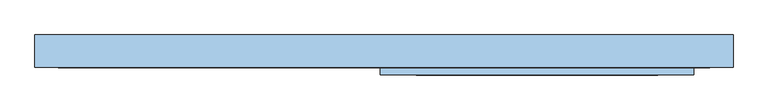
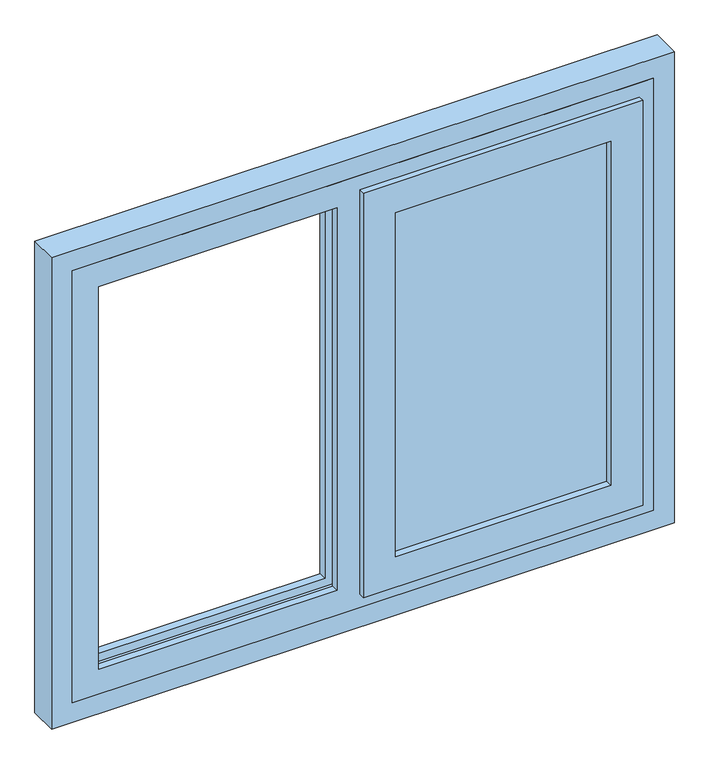
"""IFC4 building model written with IfcOpenShell, lengths in millimetres: window geometry, Окно 2-Откидное - Левое глухое - Один переплет с многокамерным стеклопакетом - 30674-99 : ОП Г1  1160-1470 (4M1-10-4M1-10-4M1) ГОСТ 30674-99."""

from ifc_helpers import new_model, si_unit, frame, origin, place, context, project, spatial, polyline, outline, extrude, faceted_brep, source, transform, mapped, element, save


def window_999542c6(model_context):
    return source(origin(), model_context, "Body", "SolidModel", [
        extrude(outline(polyline([(942.0, 608.0), (1858.0, 608.0), (1858.0, 49.0), (942.0, 49.0), (942.0, 608.0)]), holes=[polyline([(1843.0, 593.0), (957.0, 593.0), (957.0, 64.0), (1843.0, 64.0), (1843.0, 593.0)])]), frame((0.0, 25.0, 0.0), z_axis=(0.0, 1.0, 0.0), x_axis=(0.0, 0.0, 1.0)), (0.0, 0.0, 1.0), 10.0),
        extrude(outline(polyline([(942.0, 608.0), (1858.0, 608.0), (1858.0, 49.0), (942.0, 49.0), (942.0, 608.0)]), holes=[polyline([(1843.0, 593.0), (957.0, 593.0), (957.0, 64.0), (1843.0, 64.0), (1843.0, 593.0)])]), frame((0.0, 11.0, 0.0), z_axis=(0.0, 1.0, 0.0), x_axis=(0.0, 0.0, 1.0)), (0.0, 0.0, 1.0), 10.0),
        extrude(outline(polyline([(49.0, 25.0), (608.0, 25.0), (608.0, 21.0), (49.0, 21.0), (49.0, 25.0)])), frame((0.0, 0.0, 942.0), z_axis=(0.0, 0.0, 1.0), x_axis=(1.0, 0.0, 0.0)), (0.0, 0.0, 1.0), 916.0),
        extrude(outline(polyline([(49.0, 39.0), (608.0, 39.0), (608.0, 35.0), (49.0, 35.0), (49.0, 39.0)])), frame((0.0, 0.0, 942.0), z_axis=(0.0, 0.0, 1.0), x_axis=(1.0, 0.0, 0.0)), (0.0, 0.0, 1.0), 916.0),
        extrude(outline(polyline([(49.0, 11.0), (608.0, 11.0), (608.0, 7.0), (49.0, 7.0), (49.0, 11.0)])), frame((0.0, 0.0, 942.0), z_axis=(0.0, 0.0, 1.0), x_axis=(1.0, 0.0, 0.0)), (0.0, 0.0, 1.0), 916.0),
        faceted_brep([(-700.0, 5.0, 1950.0), (-700.0, 75.0, 1950.0), (-700.0, 75.0, 850.0), (-700.0, 5.0, 850.0), (700.0, 75.0, 850.0), (700.0, 75.0, 1950.0), (-637.0, 75.0, 1887.0), (-637.0, 75.0, 913.0), (-63.0, 75.0, 913.0), (-63.0, 75.0, 1887.0), (19.0, 75.0, 1887.0), (19.0, 75.0, 913.0), (637.0, 75.0, 913.0), (637.0, 75.0, 1887.0), (700.0, 5.0, 850.0), (700.0, 5.0, 1950.0), (-637.0, 5.0, 913.0), (-637.0, 5.0, 1887.0), (-63.0, 5.0, 1887.0), (-63.0, 5.0, 913.0), (0.0, 5.0, 893.0), (0.0, 5.0, 1907.0), (657.0, 5.0, 1907.0), (657.0, 5.0, 893.0), (-637.0, 23.0, 1887.0), (-637.0, 23.0, 913.0), (-63.0, 23.0, 913.0), (-657.0, 23.0, 893.0), (-657.0, 23.0, 1907.0), (-43.0, 23.0, 1907.0), (-43.0, 23.0, 893.0), (-63.0, 23.0, 1887.0), (-657.0, 55.0, 1907.0), (-657.0, 55.0, 893.0), (-43.0, 55.0, 893.0), (-43.0, 55.0, 1907.0), (-637.0, 55.0, 913.0), (-637.0, 55.0, 1887.0), (-63.0, 55.0, 1887.0), (-63.0, 55.0, 913.0), (0.0, 61.0, 893.0), (0.0, 61.0, 1907.0), (657.0, 61.0, 893.0), (657.0, 61.0, 1907.0), (19.0, 61.0, 913.0), (19.0, 61.0, 1887.0), (637.0, 61.0, 1887.0), (637.0, 61.0, 913.0)], [[[0, 1, 2, 3]], [[4, 2, 1, 5], [6, 7, 8, 9], [10, 11, 12, 13]], [[3, 2, 4, 14]], [[15, 0, 3, 14], [16, 17, 18, 19], [20, 21, 22, 23]], [[24, 17, 16, 25]], [[25, 16, 19, 26]], [[27, 28, 29, 30], [24, 25, 26, 31]], [[32, 28, 27, 33]], [[33, 27, 30, 34]], [[32, 33, 34, 35], [36, 37, 38, 39]], [[6, 37, 36, 7]], [[7, 36, 39, 8]], [[15, 14, 4, 5]], [[26, 19, 18, 31]], [[34, 30, 29, 35]], [[8, 39, 38, 9]], [[40, 41, 21, 20]], [[42, 43, 41, 40], [44, 45, 46, 47]], [[20, 23, 42, 40]], [[11, 10, 45, 44]], [[47, 12, 11, 44]], [[46, 13, 12, 47]], [[43, 42, 23, 22]], [[5, 1, 0, 15]], [[17, 24, 31, 18]], [[28, 32, 35, 29]], [[37, 6, 9, 38]], [[13, 46, 45, 10]], [[41, 43, 22, 21]]]),
        faceted_brep([(69.0, 59.0, 1838.0), (69.0, 39.0, 1838.0), (69.0, 39.0, 962.0), (69.0, 59.0, 962.0), (49.0, 39.0, 942.0), (608.0, 39.0, 942.0), (608.0, 39.0, 1858.0), (49.0, 39.0, 1858.0), (588.0, 39.0, 1838.0), (588.0, 39.0, 962.0), (588.0, 59.0, 962.0), (12.0, 59.0, 1895.0), (645.0, 59.0, 1895.0), (645.0, 59.0, 905.0), (12.0, 59.0, 905.0), (588.0, 59.0, 1838.0), (12.0, 3.0, 1895.0), (12.0, 3.0, 905.0), (645.0, 3.0, 905.0), (-8.0, 3.0, 1915.0), (665.0, 3.0, 1915.0), (665.0, 3.0, 885.0), (-8.0, 3.0, 885.0), (645.0, 3.0, 1895.0), (-8.0, -11.0, 1915.0), (-8.0, -11.0, 885.0), (665.0, -11.0, 885.0), (665.0, -11.0, 1915.0), (69.0, -11.0, 1838.0), (588.0, -11.0, 1838.0), (588.0, -11.0, 962.0), (69.0, -11.0, 962.0), (69.0, 7.0, 1838.0), (69.0, 7.0, 962.0), (588.0, 7.0, 962.0), (49.0, 7.0, 1858.0), (608.0, 7.0, 1858.0), (608.0, 7.0, 942.0), (49.0, 7.0, 942.0), (588.0, 7.0, 1838.0)], [[[0, 1, 2, 3]], [[4, 5, 6, 7], [1, 8, 9, 2]], [[3, 2, 9, 10]], [[11, 12, 13, 14], [3, 10, 15, 0]], [[16, 11, 14, 17]], [[17, 14, 13, 18]], [[19, 20, 21, 22], [17, 18, 23, 16]], [[24, 19, 22, 25]], [[25, 22, 21, 26]], [[25, 26, 27, 24], [28, 29, 30, 31]], [[32, 28, 31, 33]], [[33, 31, 30, 34]], [[35, 36, 37, 38], [33, 34, 39, 32]], [[7, 35, 38, 4]], [[4, 38, 37, 5]], [[10, 9, 8, 15]], [[18, 13, 12, 23]], [[26, 21, 20, 27]], [[34, 30, 29, 39]], [[5, 37, 36, 6]], [[15, 8, 1, 0]], [[23, 12, 11, 16]], [[27, 20, 19, 24]], [[39, 29, 28, 32]], [[6, 36, 35, 7]]]),
        extrude(outline(polyline([(800.0, -750.0), (800.0, 750.0), (2000.0, 750.0), (2000.0, -750.0), (800.0, -750.0)]), holes=[polyline([(1950.0, -700.0), (1950.0, 700.0), (850.0, 700.0), (850.0, -700.0), (1950.0, -700.0)])]), frame((0.0, 5.0, 0.0), z_axis=(0.0, 1.0, 0.0), x_axis=(0.0, 0.0, 1.0)), (0.0, 0.0, 1.0), 70.0),
    ])


if __name__ == "__main__":
    model = new_model("IFC4")
    model_context = context("Model", 3, world=origin())
    ifc_project = project(units=[si_unit("LENGTHUNIT", "METRE", prefix="MILLI")], contexts=[model_context])
    site = spatial("IfcSite", under=ifc_project)
    building = spatial("IfcBuilding", under=site)
    placement = place(None, origin())
    window_shape = window_999542c6(model_context)
    element("IfcWindow", 1, ObjectType="Окно 2-Откидное - Левое глухое - Один переплет с многокамерным стеклопакетом - 30674-99 : ОП Г1  1160-1470 (4M1-10-4M1-10-4M1) ГОСТ 30674-99", at=placement, inside=building, context=model_context, shape_type="MappedRepresentation", body=[
        mapped(window_shape, transform((0.0, 0.0, 0.0), x_axis=(1.0, 0.0, 0.0), y_axis=(0.0, 1.0, 0.0), z_axis=(0.0, 0.0, 1.0))),
    ])
    save(model, "model.ifc")

# Revit data of these elements
# Type "Окно 2-Откидное - Левое глухое - Один переплет с многокамерным стеклопакетом - 30674-99 : ОП Г1  1160-1470 (4M1-10-4M1-10-4M1) ГОСТ 30674-99"
#   Type Mark = "107"
#   Description = "ОП Г1  1200-1400 (4M1-10-4M1-10-4M1) ГОСТ 30674-99"
#   Вставка окна [instance default] = 0 mm
#   Visual Light Transmittance = 0.9
#   Solar Heat Gain Coefficient = 0.78
#   Ширина переплета 1 = 77 mm
#   Rough Width = 1500 mm
#   Rough Height = 1200 mm
#   Height = 1100 mm
#   Толщина_Тепл_Изоляции = 50 mm
#   Heat Transfer Coefficient (U) = 3.6886 W/(m²·K)
#   G = 32 mm
#   Ширина каркаса = 63 mm
#   Высота подоконника по умолчанию = 800 mm
#   Width = 1400 mm
#   Трехкамерный стеклопакет = yes
#   Двухкамерный стеклопакет = no
#   Переплет = Деревянный переплет
#   Тепловая изоляция = Тепловая изоляция
#   Оконное стекло = Стекло
#   Кадр = Деревянный каркас
#   Construction Type Id = ""
#   Wall Closure = (empty or 0)
#   Analytic Construction = (empty or 0)
# Element 1 (IfcWindow, "Окно 2-Откидное - Левое глухое - Один переплет с многокамерным стеклопакетом - 30674-99 : ОП Г1  1160-1470 (4M1-10-4M1-10-4M1) ГОСТ 30674-99")
#   Materials on its faces: "Деревянный каркас", "Деревянный переплет", "Алюминий", "Стекло", "Тепловая изоляция"
# Materials
#   "Деревянный переплет": class "Древесина", colour RGB 224 176 126, transparency 0, Cost = 0
#   "Тепловая изоляция": class "Пластмасса", colour RGB 185 154 119, transparency 0, Cost = 0
#   "Стекло": class "Стекло", colour RGB 0 0 255, transparency 0.75
#   "Деревянный каркас": class "Древесина", colour RGB 224 176 126, transparency 0, Cost = 0
#   "Алюминий": class "Металл", colour RGB 247 247 247, transparency 0
